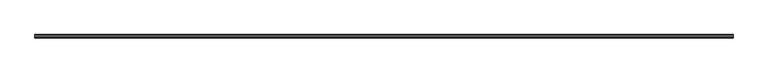
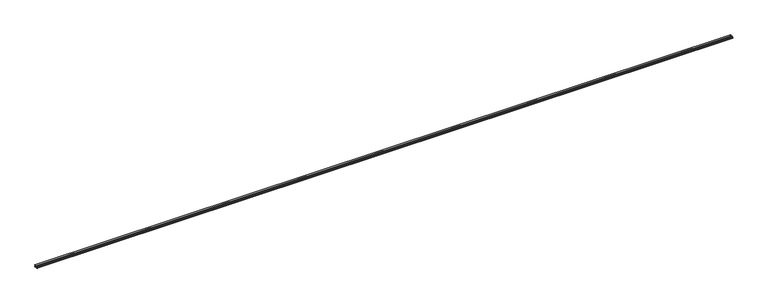
"""IFC4 building model written with IfcOpenShell, lengths in millimetres: proxy geometry, Generic Models 7:Generic Models 1:1:Generic Models 1:1 : Generic Models 7:Generic Models 1:337419:45 : Generic Models 7:Generic Models 1:1:Generic Models 1:1 : Generic Models 7:Generic Models 1:337419:306201."""

from ifc_helpers import new_model, si_unit, frame, origin, place, context, project, spatial, polyline, outline, extrude, source, transform, mapped, element, save


def generic_models_a8eaa34c(model_context):
    return source(origin(), model_context, "Body", "SweptSolid", [
        extrude(outline(polyline([(-536512.6463587, 10085.5977062), (-536511.0421571, 10086.3180886), (-536508.600138, 10088.3385088), (-536507.480634, 10090.8563718), (-536507.858781, 10093.4777811), (-536509.6754214, 10095.7926415), (-536512.6463587, 10097.4388145), (-536501.7038841, 10097.4388145), (-536502.4076536, 10095.6379157), (-536502.992597, 10091.5182603), (-536502.4076536, 10087.3986049), (-536501.7038841, 10085.5977062), (-536512.6463587, 10085.5977062)])), frame((591280.6367239, 0.0, 0.0), z_axis=(1.0, 0.0, 0.0), x_axis=(0.0, 1.0, 0.0)), (0.0, 0.0, 1.0), 4782.0596551),
        extrude(outline(polyline([(-536519.0300839, 10085.7461469), (-536522.5910207, 10086.8893847), (-536525.0552655, 10088.9494282), (-536525.9347442, 10091.5182603), (-536525.0552655, 10094.0870925), (-536522.5910207, 10096.1471359), (-536519.0300839, 10097.2903738), (-536517.053913, 10097.4388145), (-536515.0777422, 10097.2903738), (-536511.5168054, 10096.1471359), (-536509.0525606, 10094.0870925), (-536508.1730819, 10091.5182603), (-536509.0525606, 10088.9494282), (-536511.5168054, 10086.8893847), (-536515.0777422, 10085.7461469), (-536517.053913, 10085.5977062), (-536519.0300839, 10085.7461469)])), frame((591280.6367239, 0.0, 0.0), z_axis=(1.0, 0.0, 0.0), x_axis=(0.0, 1.0, 0.0)), (0.0, 0.0, 1.0), 4782.0596551),
    ])


if __name__ == "__main__":
    model = new_model("IFC4")
    model_context = context("Model", 3, world=origin())
    ifc_project = project(units=[si_unit("LENGTHUNIT", "METRE", prefix="MILLI")], contexts=[model_context])
    site = spatial("IfcSite", under=ifc_project)
    building = spatial("IfcBuilding", under=site)
    placement = place(None, origin())
    generic_models_shape = generic_models_a8eaa34c(model_context)
    element("IfcBuildingElementProxy", 1, Name="Generic Models 7:Generic Models 1:1:Generic Models 1:1 : Generic Models 7:Generic Models 1:337419:45 : Generic Models 7:Generic Models 1:1:Generic Models 1:1 : Generic Models 7:Generic Models 1:337419:306201", ObjectType="Generic Models 7:Generic Models 1:1:Generic Models 1:1 : Generic Models 7:Generic Models 1:337419:45 : Generic Models 7:Generic Models 1:1:Generic Models 1:1 : Generic Models 7:Generic Models 1:337419:306201", at=placement, inside=building, context=model_context, shape_type="MappedRepresentation", body=[
        mapped(generic_models_shape, transform((0.0, 0.0, 0.0), x_axis=(1.0, 0.0, 0.0), y_axis=(0.0, 1.0, 0.0), z_axis=(0.0, 0.0, 1.0))),
    ])
    save(model, "model.ifc")

# Revit data of these elements
# Type "Generic Models 7:Generic Models 1:1:Generic Models 1:1 : Generic Models 7:Generic Models 1:337419:45 : Generic Models 7:Generic Models 1:1:Generic Models 1:1 : Generic Models 7:Generic Models 1:337419:306201"
#   NameOverride = "Generic Models 7:Generic Models 1:1:Generic Models 1:1 : Generic Models 7:Generic Models 1:337419:306201"
#   ObjectTypeOverride = "Generic Models 1:1 : Generic Models 7:Generic Models 1:337419"
#   Reference = "Generic Models 1"
#   Tag = "306201"
# Element 1 (IfcBuildingElementProxy, "Generic Models 7:Generic Models 1:1:Generic Models 1:1 : Generic Models 7:Generic Models 1:337419:45 : Generic Models 7:Generic Models 1:1:Generic Models 1:1 : Generic Models 7:Generic Models 1:337419:306201")
#   Materials on its faces: "SEMI-RIGID EPOXY SEALANT W/ BACKROD (REMOVE TEMP. JOINT FORM)"
# Materials
#   "SEMI-RIGID EPOXY SEALANT W/ BACKROD (REMOVE TEMP. JOINT FORM)": class "Unassigned", colour RGB 120 120 120, transparency 0, Cost = 0
